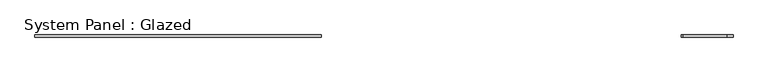
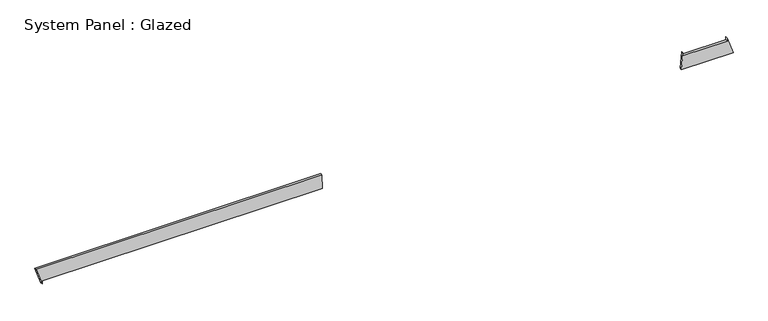
"""IFC4 building model written with IfcOpenShell, lengths in millimetres: plate geometry, System Panel : Glazed."""

from ifc_helpers import new_model, si_unit, frame, origin, place, context, project, spatial, polyline, outline, extrude, source, transform, mapped, element, save


def system_panel_glazed_58890ada(model_context):
    return source(origin(), model_context, "Body", "SweptSolid", [
        extrude(outline(polyline([(35.3553391, 3429.7598415), (35.3553391, 4028.0476561), (235.7077234, 3959.2529397), (200.3523843, 3959.2532528), (200.3478461, 3446.6577103), (235.7031851, 3446.6573973), (35.3553391, 3429.7598415)])), frame((0.0, -49.5, 0.0), z_axis=(0.0, 1.0, 0.0), x_axis=(0.0, 0.0, 1.0)), (0.0, 0.0, 1.0), 25.0),
        extrude(outline(polyline([(0.0, -3959.0814895), (35.3553391, -3959.0814895), (35.3553391, -721.6679227), (200.3109163, -724.5894165), (200.2816694, -4028.0476561), (0.0, -3959.0814895)])), frame((0.0, -49.5, 0.0), z_axis=(0.0, 1.0, 0.0), x_axis=(0.0, 0.0, 1.0)), (0.0, 0.0, 1.0), 25.0),
    ])


if __name__ == "__main__":
    model = new_model("IFC4")
    model_context = context("Model", 3, world=origin())
    ifc_project = project(units=[si_unit("LENGTHUNIT", "METRE", prefix="MILLI")], contexts=[model_context])
    site = spatial("IfcSite", under=ifc_project)
    building = spatial("IfcBuilding", under=site)
    placement = place(None, origin())
    system_panel_glazed_shape = system_panel_glazed_58890ada(model_context)
    element("IfcPlate", 1, ObjectType="System Panel : Glazed", at=placement, inside=building, context=model_context, shape_type="MappedRepresentation", body=[
        mapped(system_panel_glazed_shape, transform((0.0, 0.0, 0.0), x_axis=(1.0, 0.0, 0.0), y_axis=(0.0, 1.0, 0.0), z_axis=(0.0, 0.0, 1.0))),
    ])
    save(model, "model.ifc")

# Revit data of these elements
# Element 1 (IfcPlate, "System Panel : Glazed")
#   Materials on its faces: "Glass"
# Materials
#   "Glass": class "Glass", colour RGB 218 227 224, transparency 0.85, Description = "Soda Lime Glass", Cost = 0
